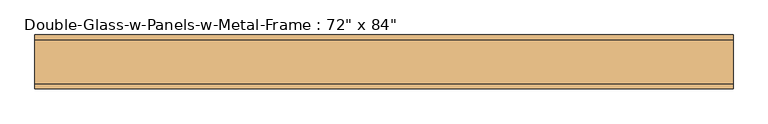
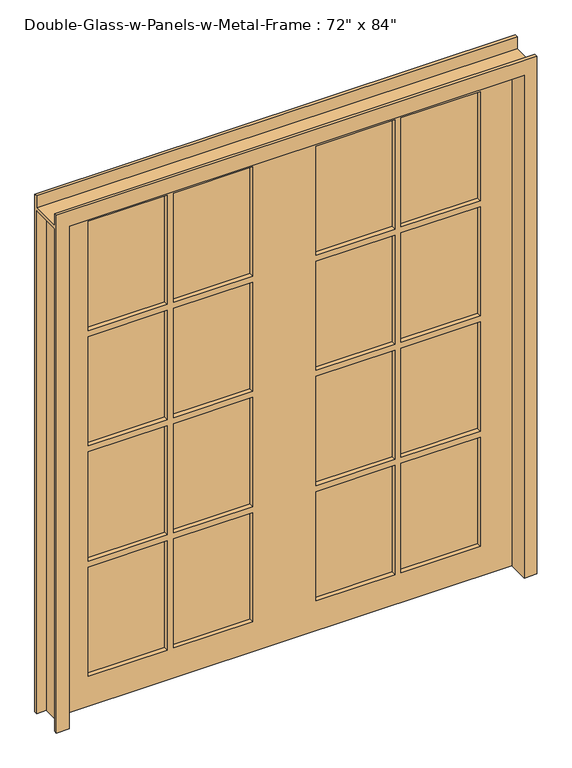
"""IFC4 building model written with IfcOpenShell, lengths in millimetres: door geometry."""

import ifcopenshell
import ifcopenshell.guid

model = None  # the IFC model being written
_history = None  # IfcOwnerHistory: only IFC2X3 demands one
_inside = {}  # id of a spatial element -> (the spatial element, [elements in it])
_under = {}  # id of a project, library or spatial element -> (it, [spatial elements below it])
_declared = {}  # id of a project -> (the project, [libraries it declares])
_typed = {}  # id of a type object -> (the type object, [elements of that type])
_made_of = {}  # id of a material, layer set ... -> (it, [elements and type objects made of it])


def new_model(schema):
    """Start an empty IFC model of exactly this schema.

    Asked for "IFC4X3", IfcOpenShell would pick the latest addendum, in which some entities
    have other attributes; the version numbers below select the first issue.
    IFC2X3 requires an IfcOwnerHistory on every rooted entity: one is made here for all.
    """
    global model, _history
    if schema == "IFC4X3":
        model = ifcopenshell.file(schema_version=(4, 3, 0, 0))
    else:
        model = ifcopenshell.file(schema=schema)
    _inside.clear()
    _under.clear()
    _declared.clear()
    _typed.clear()
    _made_of.clear()
    _history = None
    if model.schema == "IFC2X3":
        org = make("IfcOrganization", Name="unknown")
        user = make(
            "IfcPersonAndOrganization",
            ThePerson=make("IfcPerson", FamilyName="unknown"),
            TheOrganization=org,
        )
        app = make(
            "IfcApplication",
            ApplicationDeveloper=org,
            Version="unknown",
            ApplicationFullName="unknown",
            ApplicationIdentifier="unknown",
        )
        _history = make(
            "IfcOwnerHistory",
            OwningUser=user,
            OwningApplication=app,
            ChangeAction="ADDED",
            CreationDate=0,
        )
    return model


def make(cls, **values):
    """One entity of the class cls with the attributes given. An attribute that is None is left unset."""
    return model.create_entity(
        cls, **{name: value for name, value in values.items() if value is not None}
    )


def rooted(cls, **values):
    """An entity with a GlobalId (a new one), such as an element, a storey or a relation."""
    return make(cls, GlobalId=ifcopenshell.guid.new(), OwnerHistory=_history, **values)


def si_unit(unit_type, name, prefix=None):
    """IfcSIUnit, for example si_unit("LENGTHUNIT", "METRE", prefix="MILLI")."""
    return make("IfcSIUnit", UnitType=unit_type, Prefix=prefix, Name=name)


def assignment(units):
    """IfcUnitAssignment: the units of a project."""
    return None if units is None else make("IfcUnitAssignment", Units=units)


def point(xyz):
    """IfcCartesianPoint."""
    return None if xyz is None else make("IfcCartesianPoint", Coordinates=xyz)


def direction(xyz):
    """IfcDirection."""
    return None if xyz is None else make("IfcDirection", DirectionRatios=xyz)


def frame(location, z_axis=None, x_axis=None):
    """IfcAxis2Placement3D, a coordinate frame: its origin and axes. An axis left out is left unset."""
    return make(
        "IfcAxis2Placement3D",
        Location=point(location),
        Axis=direction(z_axis),
        RefDirection=direction(x_axis),
    )


def origin():
    """The frame at (0, 0, 0) with its axes left unset."""
    return frame((0.0, 0.0, 0.0))


def place(relative_to, where):
    """IfcLocalPlacement: puts the frame where relative to a parent placement (None: the world)."""
    return make(
        "IfcLocalPlacement", PlacementRelTo=relative_to, RelativePlacement=where
    )


def context(
    kind, dimensions, precision=None, world=None, true_north=None, identifier=None
):
    """IfcGeometricRepresentationContext, for example the 3D "Model" context."""
    return make(
        "IfcGeometricRepresentationContext",
        ContextIdentifier=identifier,
        ContextType=kind,
        CoordinateSpaceDimension=dimensions,
        Precision=precision,
        WorldCoordinateSystem=world,
        TrueNorth=true_north,
    )


def project(units=None, contexts=None):
    """IfcProject with its units and contexts."""
    return rooted(
        "IfcProject",
        Name="project",
        RepresentationContexts=contexts,
        UnitsInContext=assignment(units),
    )


def spatial(cls, under=None, at=None, **own):
    """A site, building, storey or space (cls), placed at a placement, below another one or the project."""
    s = rooted(cls, ObjectPlacement=at, **own)
    if under is not None:
        _under.setdefault(under.id(), (under, []))[1].append(s)
    return s


def polyline(points):
    """IfcPolyline through the points."""
    return make("IfcPolyline", Points=[point(p) for p in points])


def outline(outer, holes=None, kind="AREA"):
    """IfcArbitraryClosedProfileDef: a profile drawn as a closed curve; with holes, ...WithVoids."""
    if holes is None:
        return make("IfcArbitraryClosedProfileDef", ProfileType=kind, OuterCurve=outer)
    return make(
        "IfcArbitraryProfileDefWithVoids",
        ProfileType=kind,
        OuterCurve=outer,
        InnerCurves=holes,
    )


def extrude(swept, where, along, depth):
    """IfcExtrudedAreaSolid: the profile swept, set in the frame where, extruded along a direction by depth."""
    return make(
        "IfcExtrudedAreaSolid",
        SweptArea=swept,
        Position=where,
        ExtrudedDirection=direction(along),
        Depth=depth,
    )


def faces_of(points, faces, orient=None, outer=None):
    """IfcFace entities. A face is a list of loops; a loop is a list of indices into points, from 0.

    orient and outer hold one flag for each loop. By default every Orientation is true, the
    first loop of a face is its IfcFaceOuterBound and the others are IfcFaceBound.
    """
    made = []
    for i, loops in enumerate(faces):
        bounds = []
        for j, loop in enumerate(loops):
            is_outer = j == 0 if outer is None else outer[i][j]
            bounds.append(
                make(
                    "IfcFaceOuterBound" if is_outer else "IfcFaceBound",
                    Bound=make("IfcPolyLoop", Polygon=[points[k] for k in loop]),
                    Orientation=True if orient is None else orient[i][j],
                )
            )
        made.append(make("IfcFace", Bounds=bounds))
    return made


def faceted_brep(points, faces, orient=None, outer=None, voids=None):
    """IfcFacetedBrep: a solid bounded by flat faces; with voids (closed shells), ...WithVoids."""
    shared = [point(p) for p in points]
    hull = make("IfcClosedShell", CfsFaces=faces_of(shared, faces, orient, outer))
    if voids is None:
        return make("IfcFacetedBrep", Outer=hull)
    return make(
        "IfcFacetedBrepWithVoids",
        Outer=hull,
        Voids=[
            make(cls, CfsFaces=faces_of(shared, fs, o, b)) for cls, fs, o, b in voids
        ],
    )


def shape(context_of_items, identifier, shape_type, items):
    """IfcShapeRepresentation: the items that make up one representation, for example the "Body"."""
    return make(
        "IfcShapeRepresentation",
        ContextOfItems=context_of_items,
        RepresentationIdentifier=identifier,
        RepresentationType=shape_type,
        Items=items,
    )


def source(mapping_origin, context_of_items, identifier, shape_type, items):
    """IfcRepresentationMap: a shape defined once, which mapped items show again and again."""
    return make(
        "IfcRepresentationMap",
        MappingOrigin=mapping_origin,
        MappedRepresentation=shape(context_of_items, identifier, shape_type, items),
    )


def transform(
    local_origin,
    x_axis=None,
    y_axis=None,
    z_axis=None,
    scale=None,
    scale2=None,
    scale3=None,
    uniform=True,
):
    """IfcCartesianTransformationOperator3D, or its non-uniform kind. x_axis, y_axis, z_axis: its Axis1, 2, 3."""
    if uniform:
        return make(
            "IfcCartesianTransformationOperator3D",
            Axis1=direction(x_axis),
            Axis2=direction(y_axis),
            LocalOrigin=point(local_origin),
            Scale=scale,
            Axis3=direction(z_axis),
        )
    return make(
        "IfcCartesianTransformationOperator3DnonUniform",
        Axis1=direction(x_axis),
        Axis2=direction(y_axis),
        LocalOrigin=point(local_origin),
        Scale=scale,
        Axis3=direction(z_axis),
        Scale2=scale2,
        Scale3=scale3,
    )


def mapped(mapping_source, mapping_target):
    """IfcMappedItem: shows the shape of a source again, moved by a transform."""
    return make(
        "IfcMappedItem", MappingSource=mapping_source, MappingTarget=mapping_target
    )


def made_of(thing, what):
    """Note that an element or type object is made of a material, layer set ...; save() writes the relation."""
    if what is not None:
        _made_of.setdefault(what.id(), (what, []))[1].append(thing)
    return thing


def element(
    cls,
    number,
    at=None,
    inside=None,
    cuts=None,
    type_object=None,
    material=None,
    context=None,
    identifier="Body",
    shape_type=None,
    held_by="IfcProductDefinitionShape",
    body=None,
    shapes=None,
    **own,
):
    """One element of the class cls, such as IfcWall. Its Tag is "e" and its number.

    at: its placement. inside: the storey or other place that contains it. cuts: it is an
    opening in that element (IfcRelVoidsElement). A single representation is given by context,
    identifier, shape_type and body (its items); several are given by shapes. held_by: the class
    of the entity that holds the representations. save() writes the other relations.
    """
    e = rooted(cls, Tag="e%d" % number, ObjectPlacement=at, **own)
    if body is not None:
        shapes = [shape(context, identifier, shape_type, body)]
    if shapes is not None:
        e.Representation = make(held_by, Representations=shapes)
    if inside is not None:
        _inside.setdefault(inside.id(), (inside, []))[1].append(e)
    if cuts is not None:
        rooted(
            "IfcRelVoidsElement", RelatingBuildingElement=cuts, RelatedOpeningElement=e
        )
    if type_object is not None:
        _typed.setdefault(type_object.id(), (type_object, []))[1].append(e)
    return made_of(e, material)


def aggregate(whole, parts):
    """IfcRelAggregates: a whole, such as a stair, and the parts it consists of."""
    return rooted("IfcRelAggregates", RelatingObject=whole, RelatedObjects=parts)


def save(model, path):
    """Write the relations noted so far, then the file.

    IfcRelAggregates (storeys below a building ...), IfcRelContainedInSpatialStructure (elements
    in a storey), IfcRelDefinesByType, IfcRelAssociatesMaterial and IfcRelDeclares: one each for
    every whole, place, type object, material and project.
    """
    for whole, parts in _under.values():
        aggregate(whole, parts)
    for where, things in _inside.values():
        rooted(
            "IfcRelContainedInSpatialStructure",
            RelatedElements=things,
            RelatingStructure=where,
        )
    for kind, things in _typed.values():
        rooted("IfcRelDefinesByType", RelatedObjects=things, RelatingType=kind)
    for what, things in _made_of.values():
        rooted("IfcRelAssociatesMaterial", RelatedObjects=things, RelatingMaterial=what)
    for by, libraries in _declared.values():
        rooted("IfcRelDeclares", RelatingContext=by, RelatedDefinitions=libraries)
    model.write(path)


def door_aa07bd17(model_context):
    return source(origin(), model_context, "Body", "SolidModel", [
        extrude(outline(polyline([(469.9, 42.8625), (787.4, 42.8625), (787.4, 30.1625), (469.9, 30.1625), (469.9, 42.8625)])), frame((0.0, 0.0, 1593.85), z_axis=(0.0, 0.0, 1.0), x_axis=(1.0, 0.0, 0.0)), (0.0, 0.0, 1.0), 463.55),
        extrude(outline(polyline([(127.0, 42.8625), (444.5, 42.8625), (444.5, 30.1625), (127.0, 30.1625), (127.0, 42.8625)])), frame((0.0, 0.0, 1593.85), z_axis=(0.0, 0.0, 1.0), x_axis=(1.0, 0.0, 0.0)), (0.0, 0.0, 1.0), 463.55),
        extrude(outline(polyline([(-444.5, 42.8625), (-127.0, 42.8625), (-127.0, 30.1625), (-444.5, 30.1625), (-444.5, 42.8625)])), frame((0.0, 0.0, 1593.85), z_axis=(0.0, 0.0, 1.0), x_axis=(1.0, 0.0, 0.0)), (0.0, 0.0, 1.0), 463.55),
        extrude(outline(polyline([(-787.4, 42.8625), (-469.9, 42.8625), (-469.9, 30.1625), (-787.4, 30.1625), (-787.4, 42.8625)])), frame((0.0, 0.0, 1593.85), z_axis=(0.0, 0.0, 1.0), x_axis=(1.0, 0.0, 0.0)), (0.0, 0.0, 1.0), 463.55),
        extrude(outline(polyline([(-787.4, 42.8625), (-469.9, 42.8625), (-469.9, 30.1625), (-787.4, 30.1625), (-787.4, 42.8625)])), frame((0.0, 0.0, 1104.9), z_axis=(0.0, 0.0, 1.0), x_axis=(1.0, 0.0, 0.0)), (0.0, 0.0, 1.0), 463.55),
        extrude(outline(polyline([(-444.5, 42.8625), (-127.0, 42.8625), (-127.0, 30.1625), (-444.5, 30.1625), (-444.5, 42.8625)])), frame((0.0, 0.0, 1104.9), z_axis=(0.0, 0.0, 1.0), x_axis=(1.0, 0.0, 0.0)), (0.0, 0.0, 1.0), 463.55),
        extrude(outline(polyline([(127.0, 42.8625), (444.5, 42.8625), (444.5, 30.1625), (127.0, 30.1625), (127.0, 42.8625)])), frame((0.0, 0.0, 1104.9), z_axis=(0.0, 0.0, 1.0), x_axis=(1.0, 0.0, 0.0)), (0.0, 0.0, 1.0), 463.55),
        extrude(outline(polyline([(469.9, 42.8625), (787.4, 42.8625), (787.4, 30.1625), (469.9, 30.1625), (469.9, 42.8625)])), frame((0.0, 0.0, 1104.9), z_axis=(0.0, 0.0, 1.0), x_axis=(1.0, 0.0, 0.0)), (0.0, 0.0, 1.0), 463.55),
        extrude(outline(polyline([(469.9, 42.8625), (787.4, 42.8625), (787.4, 30.1625), (469.9, 30.1625), (469.9, 42.8625)])), frame((0.0, 0.0, 615.95), z_axis=(0.0, 0.0, 1.0), x_axis=(1.0, 0.0, 0.0)), (0.0, 0.0, 1.0), 463.55),
        extrude(outline(polyline([(127.0, 42.8625), (444.5, 42.8625), (444.5, 30.1625), (127.0, 30.1625), (127.0, 42.8625)])), frame((0.0, 0.0, 615.95), z_axis=(0.0, 0.0, 1.0), x_axis=(1.0, 0.0, 0.0)), (0.0, 0.0, 1.0), 463.55),
        extrude(outline(polyline([(-444.5, 42.8625), (-127.0, 42.8625), (-127.0, 30.1625), (-444.5, 30.1625), (-444.5, 42.8625)])), frame((0.0, 0.0, 615.95), z_axis=(0.0, 0.0, 1.0), x_axis=(1.0, 0.0, 0.0)), (0.0, 0.0, 1.0), 463.55),
        extrude(outline(polyline([(-787.4, 42.8625), (-469.9, 42.8625), (-469.9, 30.1625), (-787.4, 30.1625), (-787.4, 42.8625)])), frame((0.0, 0.0, 615.95), z_axis=(0.0, 0.0, 1.0), x_axis=(1.0, 0.0, 0.0)), (0.0, 0.0, 1.0), 463.55),
        extrude(outline(polyline([(469.9, 42.8625), (787.4, 42.8625), (787.4, 30.1625), (469.9, 30.1625), (469.9, 42.8625)])), frame((0.0, 0.0, 127.0), z_axis=(0.0, 0.0, 1.0), x_axis=(1.0, 0.0, 0.0)), (0.0, 0.0, 1.0), 463.55),
        extrude(outline(polyline([(127.0, 42.8625), (444.5, 42.8625), (444.5, 30.1625), (127.0, 30.1625), (127.0, 42.8625)])), frame((0.0, 0.0, 127.0), z_axis=(0.0, 0.0, 1.0), x_axis=(1.0, 0.0, 0.0)), (0.0, 0.0, 1.0), 463.55),
        extrude(outline(polyline([(-444.5, 42.8625), (-127.0, 42.8625), (-127.0, 30.1625), (-444.5, 30.1625), (-444.5, 42.8625)])), frame((0.0, 0.0, 127.0), z_axis=(0.0, 0.0, 1.0), x_axis=(1.0, 0.0, 0.0)), (0.0, 0.0, 1.0), 463.55),
        extrude(outline(polyline([(-787.4, 42.8625), (-469.9, 42.8625), (-469.9, 30.1625), (-787.4, 30.1625), (-787.4, 42.8625)])), frame((0.0, 0.0, 127.0), z_axis=(0.0, 0.0, 1.0), x_axis=(1.0, 0.0, 0.0)), (0.0, 0.0, 1.0), 463.55),
        extrude(outline(polyline([(2133.6, 0.0), (2133.6, -914.4), (0.0, -914.4), (0.0, 0.0), (0.0, 914.4), (2133.6, 914.4), (2133.6, 0.0)]), holes=[polyline([(2057.4, 469.9), (2057.4, 787.4), (1593.85, 787.4), (1593.85, 469.9), (2057.4, 469.9)]), polyline([(2057.4, 127.0), (2057.4, 444.5), (1593.85, 444.5), (1593.85, 127.0), (2057.4, 127.0)]), polyline([(1568.45, 469.9), (1568.45, 787.4), (1104.9, 787.4), (1104.9, 469.9), (1568.45, 469.9)]), polyline([(1568.45, 127.0), (1568.45, 444.5), (1104.9, 444.5), (1104.9, 127.0), (1568.45, 127.0)]), polyline([(1079.5, 469.9), (1079.5, 787.4), (615.95, 787.4), (615.95, 469.9), (1079.5, 469.9)]), polyline([(1079.5, 127.0), (1079.5, 444.5), (615.95, 444.5), (615.95, 127.0), (1079.5, 127.0)]), polyline([(590.55, 469.9), (590.55, 787.4), (127.0, 787.4), (127.0, 469.9), (590.55, 469.9)]), polyline([(590.55, 127.0), (590.55, 444.5), (127.0, 444.5), (127.0, 127.0), (590.55, 127.0)]), polyline([(2057.4, -444.5), (2057.4, -127.0), (1593.85, -127.0), (1593.85, -444.5), (2057.4, -444.5)]), polyline([(1568.45, -444.5), (1568.45, -127.0), (1104.9, -127.0), (1104.9, -444.5), (1568.45, -444.5)]), polyline([(1568.45, -469.9), (1104.9, -469.9), (1104.9, -787.4), (1568.45, -787.4), (1568.45, -469.9)]), polyline([(1079.5, -444.5), (1079.5, -127.0), (615.95, -127.0), (615.95, -444.5), (1079.5, -444.5)]), polyline([(1079.5, -469.9), (615.95, -469.9), (615.95, -787.4), (1079.5, -787.4), (1079.5, -469.9)]), polyline([(590.55, -444.5), (590.55, -127.0), (127.0, -127.0), (127.0, -444.5), (590.55, -444.5)]), polyline([(590.55, -787.4), (590.55, -469.9), (127.0, -469.9), (127.0, -787.4), (590.55, -787.4)]), polyline([(1593.85, -469.9), (1593.85, -787.4), (2057.4, -787.4), (2057.4, -469.9), (1593.85, -469.9)])]), frame((0.0, 11.1125, 0.0), z_axis=(0.0, 1.0, 0.0), x_axis=(0.0, 0.0, 1.0)), (0.0, 0.0, 1.0), 50.8),
        faceted_brep([(-927.1, 61.9125, 0.0), (-965.2, 61.9125, 0.0), (-965.2, 74.6125, 0.0), (-914.4, 74.6125, 0.0), (-914.4, -74.6125, 0.0), (-965.2, -74.6125, 0.0), (-965.2, -61.9125, 0.0), (-927.1, -61.9125, 0.0), (-927.1, 61.9125, 2133.6), (-965.2, 61.9125, 2133.6), (-965.2, -61.9125, 2133.6), (-965.2, -74.6125, 2197.1), (-965.2, -61.9125, 2197.1), (-965.2, -61.9125, 2146.3), (-965.2, 61.9125, 2146.3), (-965.2, 61.9125, 2197.1), (-965.2, 74.6125, 2197.1), (965.2, 74.6125, 2197.1), (965.2, 74.6125, 0.0), (914.4, 74.6125, 0.0), (914.4, 74.6125, 2133.6), (-914.4, 74.6125, 2133.6), (-914.4, -74.6125, 2133.6), (914.4, -74.6125, 2133.6), (914.4, -74.6125, 0.0), (965.2, -74.6125, 0.0), (965.2, -74.6125, 2197.1), (-927.1, -61.9125, 2133.6), (927.1, 61.9125, 0.0), (927.1, -61.9125, 0.0), (965.2, -61.9125, 0.0), (965.2, 61.9125, 0.0), (965.2, -61.9125, 2146.3), (965.2, -61.9125, 2197.1), (965.2, -61.9125, 2133.6), (965.2, 61.9125, 2133.6), (965.2, 61.9125, 2197.1), (965.2, 61.9125, 2146.3), (927.1, -61.9125, 2133.6), (927.1, 61.9125, 2133.6)], [[[0, 1, 2, 3, 4, 5, 6, 7]], [[1, 0, 8, 9]], [[2, 1, 9, 10, 6, 5, 11, 12, 13, 14, 15, 16]], [[3, 2, 16, 17, 18, 19, 20, 21]], [[4, 3, 21, 22]], [[5, 4, 22, 23, 24, 25, 26, 11]], [[7, 6, 10, 27]], [[0, 7, 27, 8]], [[19, 24, 23, 20]], [[28, 29, 30, 25, 24, 19, 18, 31]], [[32, 33, 26, 25, 30, 34, 35, 31, 18, 17, 36, 37]], [[30, 29, 38, 34]], [[28, 31, 35, 39]], [[29, 28, 39, 38]], [[33, 32, 13, 12]], [[26, 33, 12, 11]], [[10, 9, 8, 27]], [[22, 21, 20, 23]], [[35, 34, 38, 39]], [[36, 17, 16, 15]], [[37, 36, 15, 14]], [[32, 37, 14, 13]]]),
    ])


if __name__ == "__main__":
    model = new_model("IFC4")
    model_context = context("Model", 3, world=origin())
    ifc_project = project(units=[si_unit("LENGTHUNIT", "METRE", prefix="MILLI")], contexts=[model_context])
    site = spatial("IfcSite", under=ifc_project)
    building = spatial("IfcBuilding", under=site)
    placement = place(None, origin())
    door_shape = door_aa07bd17(model_context)
    element("IfcDoor", 1, ObjectType="Double-Glass-w-Panels-w-Metal-Frame : 72\" x 84\"", at=placement, inside=building, context=model_context, shape_type="MappedRepresentation", body=[
        mapped(door_shape, transform((0.0, 0.0, 0.0), x_axis=(1.0, 0.0, 0.0), y_axis=(0.0, 1.0, 0.0), z_axis=(0.0, 0.0, 1.0))),
    ])
    save(model, "model.ifc")

# Revit data of these elements
# Type "Double-Glass-w-Panels-w-Metal-Frame : 72\" x 84\""
#   Type Mark = "10"
#   Construction Type Id = "opn-d46"
#   Assembly Code = "C1020300"
#   Analytic Construction = "Metal frame, double glass door"
#   Thickness = 0' - 2"
#   Thermal Resistance (R) = 1.3794 (h·ft²·°F)/BTU
#   Half Width Neg = -3' - 2"
#   Half Width = 3' - 2"
#   Frame Width = 0' - 2"
#   Frame Thickness = 0' - 0 1/2"
#   Frame Head Heigth = 0' - 2"
#   Heat Transfer Coefficient (U) = 0.7250 BTU/(h·ft²·°F)
#   Height = 7' - 0"
#   Muntin = 0' - 1"
#   Width = 6' - 0"
#   Define Thermal Properties by = 1
#   Define Thermal Properties by = 1
#   Door Material = Aluminum Painted - Red
#   Frame Material = Aluminum Painted - Red
#   Visual Light Transmittance = 0
#   Solar Heat Gain Coefficient = 0
#   Function = (empty or 0)
#   Wall Closure = (empty or 0)
# Element 1 (IfcDoor, "Double-Glass-w-Panels-w-Metal-Frame : 72\" x 84\"")
#   Materials on its faces: "Aluminum Painted - Red", "Glass"
# Materials
#   "Aluminum Painted - Red": class "Metal", colour RGB 255 0 0, transparency 0, Description = "Aluminum 6061", Cost = 0
#   "Glass": class "Glass", colour RGB 0 128 192, transparency 0.75, Description = "Soda Lime Glass", Cost = 0
